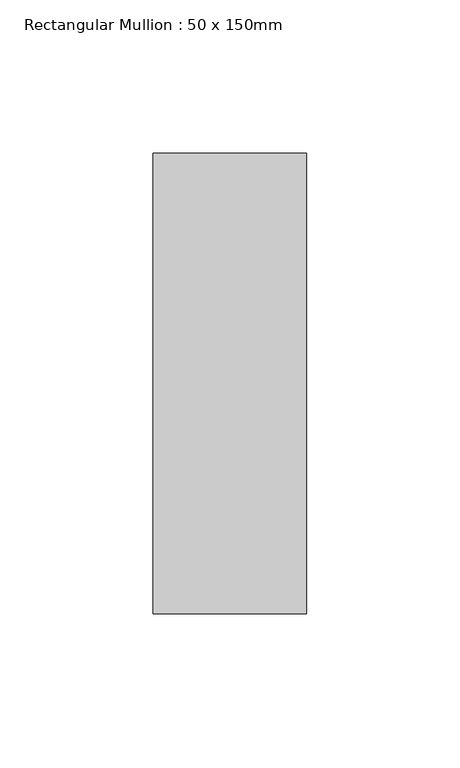
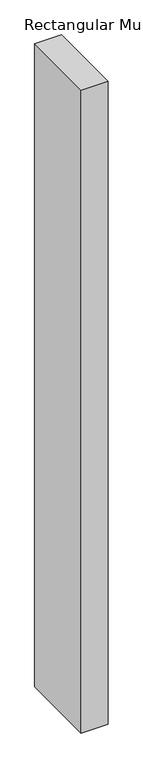
"""IFC4 building model written with IfcOpenShell, lengths in millimetres: member geometry, Rectangular Mullion : 50 x 150mm."""

import ifcopenshell
import ifcopenshell.guid

model = None  # the IFC model being written
_history = None  # IfcOwnerHistory: only IFC2X3 demands one
_inside = {}  # id of a spatial element -> (the spatial element, [elements in it])
_under = {}  # id of a project, library or spatial element -> (it, [spatial elements below it])
_declared = {}  # id of a project -> (the project, [libraries it declares])
_typed = {}  # id of a type object -> (the type object, [elements of that type])
_made_of = {}  # id of a material, layer set ... -> (it, [elements and type objects made of it])


def new_model(schema):
    """Start an empty IFC model of exactly this schema.

    Asked for "IFC4X3", IfcOpenShell would pick the latest addendum, in which some entities
    have other attributes; the version numbers below select the first issue.
    IFC2X3 requires an IfcOwnerHistory on every rooted entity: one is made here for all.
    """
    global model, _history
    if schema == "IFC4X3":
        model = ifcopenshell.file(schema_version=(4, 3, 0, 0))
    else:
        model = ifcopenshell.file(schema=schema)
    _inside.clear()
    _under.clear()
    _declared.clear()
    _typed.clear()
    _made_of.clear()
    _history = None
    if model.schema == "IFC2X3":
        org = make("IfcOrganization", Name="unknown")
        user = make(
            "IfcPersonAndOrganization",
            ThePerson=make("IfcPerson", FamilyName="unknown"),
            TheOrganization=org,
        )
        app = make(
            "IfcApplication",
            ApplicationDeveloper=org,
            Version="unknown",
            ApplicationFullName="unknown",
            ApplicationIdentifier="unknown",
        )
        _history = make(
            "IfcOwnerHistory",
            OwningUser=user,
            OwningApplication=app,
            ChangeAction="ADDED",
            CreationDate=0,
        )
    return model


def make(cls, **values):
    """One entity of the class cls with the attributes given. An attribute that is None is left unset."""
    return model.create_entity(
        cls, **{name: value for name, value in values.items() if value is not None}
    )


def rooted(cls, **values):
    """An entity with a GlobalId (a new one), such as an element, a storey or a relation."""
    return make(cls, GlobalId=ifcopenshell.guid.new(), OwnerHistory=_history, **values)


def si_unit(unit_type, name, prefix=None):
    """IfcSIUnit, for example si_unit("LENGTHUNIT", "METRE", prefix="MILLI")."""
    return make("IfcSIUnit", UnitType=unit_type, Prefix=prefix, Name=name)


def assignment(units):
    """IfcUnitAssignment: the units of a project."""
    return None if units is None else make("IfcUnitAssignment", Units=units)


def point(xyz):
    """IfcCartesianPoint."""
    return None if xyz is None else make("IfcCartesianPoint", Coordinates=xyz)


def direction(xyz):
    """IfcDirection."""
    return None if xyz is None else make("IfcDirection", DirectionRatios=xyz)


def frame(location, z_axis=None, x_axis=None):
    """IfcAxis2Placement3D, a coordinate frame: its origin and axes. An axis left out is left unset."""
    return make(
        "IfcAxis2Placement3D",
        Location=point(location),
        Axis=direction(z_axis),
        RefDirection=direction(x_axis),
    )


def origin():
    """The frame at (0, 0, 0) with its axes left unset."""
    return frame((0.0, 0.0, 0.0))


def place(relative_to, where):
    """IfcLocalPlacement: puts the frame where relative to a parent placement (None: the world)."""
    return make(
        "IfcLocalPlacement", PlacementRelTo=relative_to, RelativePlacement=where
    )


def context(
    kind, dimensions, precision=None, world=None, true_north=None, identifier=None
):
    """IfcGeometricRepresentationContext, for example the 3D "Model" context."""
    return make(
        "IfcGeometricRepresentationContext",
        ContextIdentifier=identifier,
        ContextType=kind,
        CoordinateSpaceDimension=dimensions,
        Precision=precision,
        WorldCoordinateSystem=world,
        TrueNorth=true_north,
    )


def project(units=None, contexts=None):
    """IfcProject with its units and contexts."""
    return rooted(
        "IfcProject",
        Name="project",
        RepresentationContexts=contexts,
        UnitsInContext=assignment(units),
    )


def spatial(cls, under=None, at=None, **own):
    """A site, building, storey or space (cls), placed at a placement, below another one or the project."""
    s = rooted(cls, ObjectPlacement=at, **own)
    if under is not None:
        _under.setdefault(under.id(), (under, []))[1].append(s)
    return s


def polyline(points):
    """IfcPolyline through the points."""
    return make("IfcPolyline", Points=[point(p) for p in points])


def outline(outer, holes=None, kind="AREA"):
    """IfcArbitraryClosedProfileDef: a profile drawn as a closed curve; with holes, ...WithVoids."""
    if holes is None:
        return make("IfcArbitraryClosedProfileDef", ProfileType=kind, OuterCurve=outer)
    return make(
        "IfcArbitraryProfileDefWithVoids",
        ProfileType=kind,
        OuterCurve=outer,
        InnerCurves=holes,
    )


def extrude(swept, where, along, depth):
    """IfcExtrudedAreaSolid: the profile swept, set in the frame where, extruded along a direction by depth."""
    return make(
        "IfcExtrudedAreaSolid",
        SweptArea=swept,
        Position=where,
        ExtrudedDirection=direction(along),
        Depth=depth,
    )


def shape(context_of_items, identifier, shape_type, items):
    """IfcShapeRepresentation: the items that make up one representation, for example the "Body"."""
    return make(
        "IfcShapeRepresentation",
        ContextOfItems=context_of_items,
        RepresentationIdentifier=identifier,
        RepresentationType=shape_type,
        Items=items,
    )


def source(mapping_origin, context_of_items, identifier, shape_type, items):
    """IfcRepresentationMap: a shape defined once, which mapped items show again and again."""
    return make(
        "IfcRepresentationMap",
        MappingOrigin=mapping_origin,
        MappedRepresentation=shape(context_of_items, identifier, shape_type, items),
    )


def transform(
    local_origin,
    x_axis=None,
    y_axis=None,
    z_axis=None,
    scale=None,
    scale2=None,
    scale3=None,
    uniform=True,
):
    """IfcCartesianTransformationOperator3D, or its non-uniform kind. x_axis, y_axis, z_axis: its Axis1, 2, 3."""
    if uniform:
        return make(
            "IfcCartesianTransformationOperator3D",
            Axis1=direction(x_axis),
            Axis2=direction(y_axis),
            LocalOrigin=point(local_origin),
            Scale=scale,
            Axis3=direction(z_axis),
        )
    return make(
        "IfcCartesianTransformationOperator3DnonUniform",
        Axis1=direction(x_axis),
        Axis2=direction(y_axis),
        LocalOrigin=point(local_origin),
        Scale=scale,
        Axis3=direction(z_axis),
        Scale2=scale2,
        Scale3=scale3,
    )


def mapped(mapping_source, mapping_target):
    """IfcMappedItem: shows the shape of a source again, moved by a transform."""
    return make(
        "IfcMappedItem", MappingSource=mapping_source, MappingTarget=mapping_target
    )


def made_of(thing, what):
    """Note that an element or type object is made of a material, layer set ...; save() writes the relation."""
    if what is not None:
        _made_of.setdefault(what.id(), (what, []))[1].append(thing)
    return thing


def element(
    cls,
    number,
    at=None,
    inside=None,
    cuts=None,
    type_object=None,
    material=None,
    context=None,
    identifier="Body",
    shape_type=None,
    held_by="IfcProductDefinitionShape",
    body=None,
    shapes=None,
    **own,
):
    """One element of the class cls, such as IfcWall. Its Tag is "e" and its number.

    at: its placement. inside: the storey or other place that contains it. cuts: it is an
    opening in that element (IfcRelVoidsElement). A single representation is given by context,
    identifier, shape_type and body (its items); several are given by shapes. held_by: the class
    of the entity that holds the representations. save() writes the other relations.
    """
    e = rooted(cls, Tag="e%d" % number, ObjectPlacement=at, **own)
    if body is not None:
        shapes = [shape(context, identifier, shape_type, body)]
    if shapes is not None:
        e.Representation = make(held_by, Representations=shapes)
    if inside is not None:
        _inside.setdefault(inside.id(), (inside, []))[1].append(e)
    if cuts is not None:
        rooted(
            "IfcRelVoidsElement", RelatingBuildingElement=cuts, RelatedOpeningElement=e
        )
    if type_object is not None:
        _typed.setdefault(type_object.id(), (type_object, []))[1].append(e)
    return made_of(e, material)


def aggregate(whole, parts):
    """IfcRelAggregates: a whole, such as a stair, and the parts it consists of."""
    return rooted("IfcRelAggregates", RelatingObject=whole, RelatedObjects=parts)


def save(model, path):
    """Write the relations noted so far, then the file.

    IfcRelAggregates (storeys below a building ...), IfcRelContainedInSpatialStructure (elements
    in a storey), IfcRelDefinesByType, IfcRelAssociatesMaterial and IfcRelDeclares: one each for
    every whole, place, type object, material and project.
    """
    for whole, parts in _under.values():
        aggregate(whole, parts)
    for where, things in _inside.values():
        rooted(
            "IfcRelContainedInSpatialStructure",
            RelatedElements=things,
            RelatingStructure=where,
        )
    for kind, things in _typed.values():
        rooted("IfcRelDefinesByType", RelatedObjects=things, RelatingType=kind)
    for what, things in _made_of.values():
        rooted("IfcRelAssociatesMaterial", RelatedObjects=things, RelatingMaterial=what)
    for by, libraries in _declared.values():
        rooted("IfcRelDeclares", RelatingContext=by, RelatedDefinitions=libraries)
    model.write(path)


def rectangular_mullion_50_x_150mm_97c2790d(model_context):
    return source(origin(), model_context, "Body", "SweptSolid", [
        extrude(outline(polyline([(25.0, 75.0), (25.0, -75.0), (-25.0, -75.0), (-25.0, 75.0), (25.0, 75.0)])), frame((0.0, 0.0, -1264.9999999), z_axis=(0.0, 0.0, 1.0), x_axis=(1.0, 0.0, 0.0)), (0.0, 0.0, 1.0), 1264.9999999),
    ])


if __name__ == "__main__":
    model = new_model("IFC4")
    model_context = context("Model", 3, world=origin())
    ifc_project = project(units=[si_unit("LENGTHUNIT", "METRE", prefix="MILLI")], contexts=[model_context])
    site = spatial("IfcSite", under=ifc_project)
    building = spatial("IfcBuilding", under=site)
    placement = place(None, origin())
    rectangular_mullion_50_x_150mm_shape = rectangular_mullion_50_x_150mm_97c2790d(model_context)
    element("IfcMember", 1, ObjectType="Rectangular Mullion : 50 x 150mm", at=placement, inside=building, context=model_context, shape_type="MappedRepresentation", body=[
        mapped(rectangular_mullion_50_x_150mm_shape, transform((0.0, 0.0, 0.0), x_axis=(1.0, 0.0, 0.0), y_axis=(0.0, 1.0, 0.0), z_axis=(0.0, 0.0, 1.0))),
    ])
    save(model, "model.ifc")

# Revit data of these elements
# Type "Rectangular Mullion : 50 x 150mm"
#   built-in parameter 1007304 = 0.492126 (stored number, unit not read)
#   built-in parameter 1007301 = 0.082021 (stored number, unit not read)
#   built-in parameter 1007300 = 0.082021 (stored number, unit not read)
# Element 1 (IfcMember, "Rectangular Mullion : 50 x 150mm")
#   Materials on its faces: "Aluminium"
# Materials
#   "Aluminium": class "Metal", colour RGB 247 247 247, transparency 0, Description = "Aluminium 6061", Cost = 0
